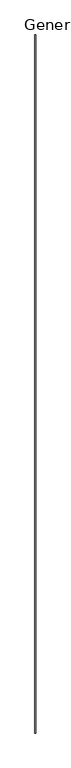
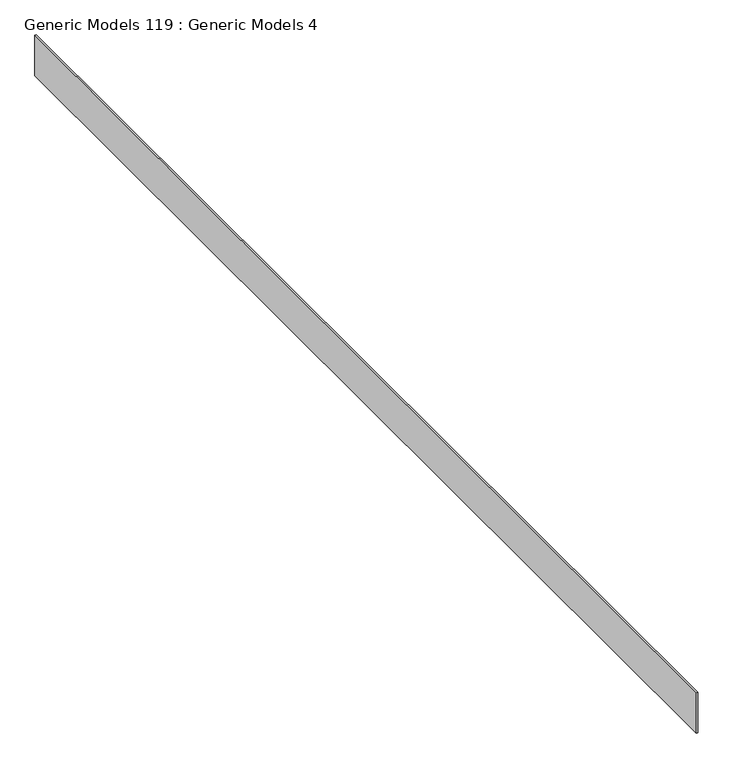
"""IFC4 building model written with IfcOpenShell, lengths in millimetres: proxy geometry, Generic Models 119 : Generic Models 4."""

from ifc_helpers import new_model, si_unit, frame, origin, place, context, project, spatial, polyline, outline, extrude, source, transform, mapped, element, save


def generic_models_119_generic_models_4_6e713bf9(model_context):
    return source(origin(), model_context, "Body", "SweptSolid", [
        extrude(outline(polyline([(7253.8514146, -6864.9230338), (7234.8014146, -6864.9230338), (7234.8014146, 11778.6769662), (7253.8514146, 11778.6769662), (7253.8514146, -6864.9230338)])), frame((0.0, 0.0, 126372.2280968), z_axis=(0.0, 0.0, 1.0), x_axis=(1.0, 0.0, 0.0)), (0.0, 0.0, 1.0), 698.1402691),
    ])


if __name__ == "__main__":
    model = new_model("IFC4")
    model_context = context("Model", 3, world=origin())
    ifc_project = project(units=[si_unit("LENGTHUNIT", "METRE", prefix="MILLI")], contexts=[model_context])
    site = spatial("IfcSite", under=ifc_project)
    building = spatial("IfcBuilding", under=site)
    placement = place(None, origin())
    generic_models_119_generic_models_4_shape = generic_models_119_generic_models_4_6e713bf9(model_context)
    element("IfcBuildingElementProxy", 1, Name="Generic Models 119 : Generic Models 4", ObjectType="Generic Models 119 : Generic Models 4", at=placement, inside=building, context=model_context, shape_type="MappedRepresentation", body=[
        mapped(generic_models_119_generic_models_4_shape, transform((0.0, 0.0, 0.0), x_axis=(1.0, 0.0, 0.0), y_axis=(0.0, 1.0, 0.0), z_axis=(0.0, 0.0, 1.0))),
    ])
    save(model, "model.ifc")

# Revit data of these elements
# Element 1 (IfcBuildingElementProxy, "Generic Models 119 : Generic Models 4")
#   Materials on its faces: "_CDX PLYWOOD - SEE STRUCT DWGs"
# Materials
#   "_CDX PLYWOOD - SEE STRUCT DWGs": class "Generic", colour RGB 98 75 74, transparency 0, Cost = 0
